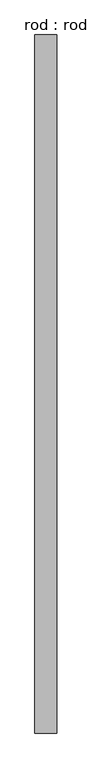
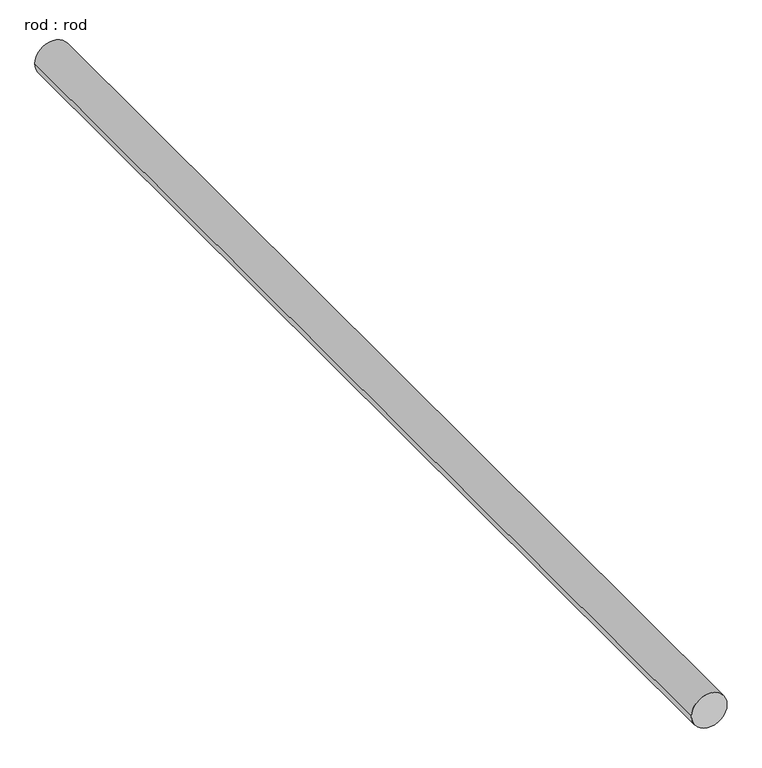
"""IFC4 building model written with IfcOpenShell, lengths in millimetres: proxy geometry, rod : rod."""

from ifc_helpers import new_model, si_unit, point, frame, frame_2d, origin, place, context, project, spatial, circle_curve, trimmed, segment, composite_curve, outline, extrude, source, transform, mapped, element, save


def rod_rod_cf6679fb(model_context):
    return source(origin(), model_context, "Body", "SweptSolid", [
        extrude(outline(composite_curve([segment(trimmed(circle_curve(frame_2d((0.0108462, 0.0)), 200.0), [point((0.0108462, 200.0))], [point((0.0108462, -200.0))], False, "CARTESIAN"), True, "CONTINUOUS"), segment(trimmed(circle_curve(frame_2d((0.0108462, 0.0)), 200.0), [point((0.0108462, -200.0))], [point((0.0108462, 200.0))], False, "CARTESIAN"), True, "CONTINUOUS")], self_intersect=False)), frame((0.0, -2279.3450834, 0.0), z_axis=(0.0, 1.0, 0.0), x_axis=(0.0, 0.0, 1.0)), (0.0, 0.0, 1.0), 12744.1473975),
    ])


if __name__ == "__main__":
    model = new_model("IFC4")
    model_context = context("Model", 3, world=origin())
    ifc_project = project(units=[si_unit("LENGTHUNIT", "METRE", prefix="MILLI")], contexts=[model_context])
    site = spatial("IfcSite", under=ifc_project)
    building = spatial("IfcBuilding", under=site)
    placement = place(None, origin())
    rod_rod_shape = rod_rod_cf6679fb(model_context)
    element("IfcBuildingElementProxy", 1, Name="rod : rod", ObjectType="rod : rod", at=placement, inside=building, context=model_context, shape_type="MappedRepresentation", body=[
        mapped(rod_rod_shape, transform((0.0, 0.0, 0.0), x_axis=(1.0, 0.0, 0.0), y_axis=(0.0, 1.0, 0.0), z_axis=(0.0, 0.0, 1.0))),
    ])
    save(model, "model.ifc")

# Revit data of these elements
# Type "rod : rod"
#   Default Elevation = 0
